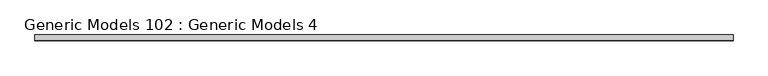
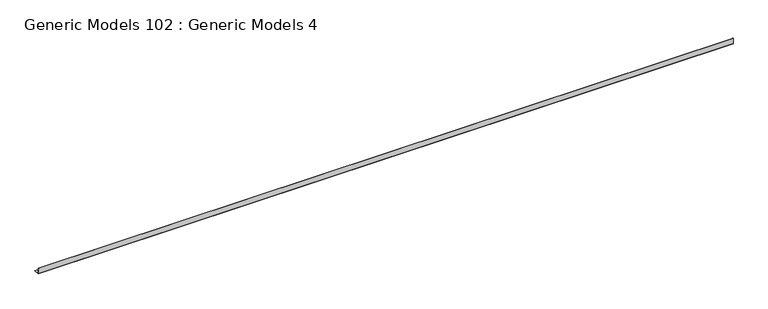
"""IFC4 building model written with IfcOpenShell, lengths in millimetres: proxy geometry, Generic Models 102 : Generic Models 4."""

import ifcopenshell
import ifcopenshell.guid

model = None  # the IFC model being written
_history = None  # IfcOwnerHistory: only IFC2X3 demands one
_inside = {}  # id of a spatial element -> (the spatial element, [elements in it])
_under = {}  # id of a project, library or spatial element -> (it, [spatial elements below it])
_declared = {}  # id of a project -> (the project, [libraries it declares])
_typed = {}  # id of a type object -> (the type object, [elements of that type])
_made_of = {}  # id of a material, layer set ... -> (it, [elements and type objects made of it])


def new_model(schema):
    """Start an empty IFC model of exactly this schema.

    Asked for "IFC4X3", IfcOpenShell would pick the latest addendum, in which some entities
    have other attributes; the version numbers below select the first issue.
    IFC2X3 requires an IfcOwnerHistory on every rooted entity: one is made here for all.
    """
    global model, _history
    if schema == "IFC4X3":
        model = ifcopenshell.file(schema_version=(4, 3, 0, 0))
    else:
        model = ifcopenshell.file(schema=schema)
    _inside.clear()
    _under.clear()
    _declared.clear()
    _typed.clear()
    _made_of.clear()
    _history = None
    if model.schema == "IFC2X3":
        org = make("IfcOrganization", Name="unknown")
        user = make(
            "IfcPersonAndOrganization",
            ThePerson=make("IfcPerson", FamilyName="unknown"),
            TheOrganization=org,
        )
        app = make(
            "IfcApplication",
            ApplicationDeveloper=org,
            Version="unknown",
            ApplicationFullName="unknown",
            ApplicationIdentifier="unknown",
        )
        _history = make(
            "IfcOwnerHistory",
            OwningUser=user,
            OwningApplication=app,
            ChangeAction="ADDED",
            CreationDate=0,
        )
    return model


def make(cls, **values):
    """One entity of the class cls with the attributes given. An attribute that is None is left unset."""
    return model.create_entity(
        cls, **{name: value for name, value in values.items() if value is not None}
    )


def rooted(cls, **values):
    """An entity with a GlobalId (a new one), such as an element, a storey or a relation."""
    return make(cls, GlobalId=ifcopenshell.guid.new(), OwnerHistory=_history, **values)


def si_unit(unit_type, name, prefix=None):
    """IfcSIUnit, for example si_unit("LENGTHUNIT", "METRE", prefix="MILLI")."""
    return make("IfcSIUnit", UnitType=unit_type, Prefix=prefix, Name=name)


def assignment(units):
    """IfcUnitAssignment: the units of a project."""
    return None if units is None else make("IfcUnitAssignment", Units=units)


def point(xyz):
    """IfcCartesianPoint."""
    return None if xyz is None else make("IfcCartesianPoint", Coordinates=xyz)


def direction(xyz):
    """IfcDirection."""
    return None if xyz is None else make("IfcDirection", DirectionRatios=xyz)


def frame(location, z_axis=None, x_axis=None):
    """IfcAxis2Placement3D, a coordinate frame: its origin and axes. An axis left out is left unset."""
    return make(
        "IfcAxis2Placement3D",
        Location=point(location),
        Axis=direction(z_axis),
        RefDirection=direction(x_axis),
    )


def origin():
    """The frame at (0, 0, 0) with its axes left unset."""
    return frame((0.0, 0.0, 0.0))


def place(relative_to, where):
    """IfcLocalPlacement: puts the frame where relative to a parent placement (None: the world)."""
    return make(
        "IfcLocalPlacement", PlacementRelTo=relative_to, RelativePlacement=where
    )


def context(
    kind, dimensions, precision=None, world=None, true_north=None, identifier=None
):
    """IfcGeometricRepresentationContext, for example the 3D "Model" context."""
    return make(
        "IfcGeometricRepresentationContext",
        ContextIdentifier=identifier,
        ContextType=kind,
        CoordinateSpaceDimension=dimensions,
        Precision=precision,
        WorldCoordinateSystem=world,
        TrueNorth=true_north,
    )


def project(units=None, contexts=None):
    """IfcProject with its units and contexts."""
    return rooted(
        "IfcProject",
        Name="project",
        RepresentationContexts=contexts,
        UnitsInContext=assignment(units),
    )


def spatial(cls, under=None, at=None, **own):
    """A site, building, storey or space (cls), placed at a placement, below another one or the project."""
    s = rooted(cls, ObjectPlacement=at, **own)
    if under is not None:
        _under.setdefault(under.id(), (under, []))[1].append(s)
    return s


def polyline(points):
    """IfcPolyline through the points."""
    return make("IfcPolyline", Points=[point(p) for p in points])


def outline(outer, holes=None, kind="AREA"):
    """IfcArbitraryClosedProfileDef: a profile drawn as a closed curve; with holes, ...WithVoids."""
    if holes is None:
        return make("IfcArbitraryClosedProfileDef", ProfileType=kind, OuterCurve=outer)
    return make(
        "IfcArbitraryProfileDefWithVoids",
        ProfileType=kind,
        OuterCurve=outer,
        InnerCurves=holes,
    )


def extrude(swept, where, along, depth):
    """IfcExtrudedAreaSolid: the profile swept, set in the frame where, extruded along a direction by depth."""
    return make(
        "IfcExtrudedAreaSolid",
        SweptArea=swept,
        Position=where,
        ExtrudedDirection=direction(along),
        Depth=depth,
    )


def shape(context_of_items, identifier, shape_type, items):
    """IfcShapeRepresentation: the items that make up one representation, for example the "Body"."""
    return make(
        "IfcShapeRepresentation",
        ContextOfItems=context_of_items,
        RepresentationIdentifier=identifier,
        RepresentationType=shape_type,
        Items=items,
    )


def source(mapping_origin, context_of_items, identifier, shape_type, items):
    """IfcRepresentationMap: a shape defined once, which mapped items show again and again."""
    return make(
        "IfcRepresentationMap",
        MappingOrigin=mapping_origin,
        MappedRepresentation=shape(context_of_items, identifier, shape_type, items),
    )


def transform(
    local_origin,
    x_axis=None,
    y_axis=None,
    z_axis=None,
    scale=None,
    scale2=None,
    scale3=None,
    uniform=True,
):
    """IfcCartesianTransformationOperator3D, or its non-uniform kind. x_axis, y_axis, z_axis: its Axis1, 2, 3."""
    if uniform:
        return make(
            "IfcCartesianTransformationOperator3D",
            Axis1=direction(x_axis),
            Axis2=direction(y_axis),
            LocalOrigin=point(local_origin),
            Scale=scale,
            Axis3=direction(z_axis),
        )
    return make(
        "IfcCartesianTransformationOperator3DnonUniform",
        Axis1=direction(x_axis),
        Axis2=direction(y_axis),
        LocalOrigin=point(local_origin),
        Scale=scale,
        Axis3=direction(z_axis),
        Scale2=scale2,
        Scale3=scale3,
    )


def mapped(mapping_source, mapping_target):
    """IfcMappedItem: shows the shape of a source again, moved by a transform."""
    return make(
        "IfcMappedItem", MappingSource=mapping_source, MappingTarget=mapping_target
    )


def made_of(thing, what):
    """Note that an element or type object is made of a material, layer set ...; save() writes the relation."""
    if what is not None:
        _made_of.setdefault(what.id(), (what, []))[1].append(thing)
    return thing


def element(
    cls,
    number,
    at=None,
    inside=None,
    cuts=None,
    type_object=None,
    material=None,
    context=None,
    identifier="Body",
    shape_type=None,
    held_by="IfcProductDefinitionShape",
    body=None,
    shapes=None,
    **own,
):
    """One element of the class cls, such as IfcWall. Its Tag is "e" and its number.

    at: its placement. inside: the storey or other place that contains it. cuts: it is an
    opening in that element (IfcRelVoidsElement). A single representation is given by context,
    identifier, shape_type and body (its items); several are given by shapes. held_by: the class
    of the entity that holds the representations. save() writes the other relations.
    """
    e = rooted(cls, Tag="e%d" % number, ObjectPlacement=at, **own)
    if body is not None:
        shapes = [shape(context, identifier, shape_type, body)]
    if shapes is not None:
        e.Representation = make(held_by, Representations=shapes)
    if inside is not None:
        _inside.setdefault(inside.id(), (inside, []))[1].append(e)
    if cuts is not None:
        rooted(
            "IfcRelVoidsElement", RelatingBuildingElement=cuts, RelatedOpeningElement=e
        )
    if type_object is not None:
        _typed.setdefault(type_object.id(), (type_object, []))[1].append(e)
    return made_of(e, material)


def aggregate(whole, parts):
    """IfcRelAggregates: a whole, such as a stair, and the parts it consists of."""
    return rooted("IfcRelAggregates", RelatingObject=whole, RelatedObjects=parts)


def save(model, path):
    """Write the relations noted so far, then the file.

    IfcRelAggregates (storeys below a building ...), IfcRelContainedInSpatialStructure (elements
    in a storey), IfcRelDefinesByType, IfcRelAssociatesMaterial and IfcRelDeclares: one each for
    every whole, place, type object, material and project.
    """
    for whole, parts in _under.values():
        aggregate(whole, parts)
    for where, things in _inside.values():
        rooted(
            "IfcRelContainedInSpatialStructure",
            RelatedElements=things,
            RelatingStructure=where,
        )
    for kind, things in _typed.values():
        rooted("IfcRelDefinesByType", RelatedObjects=things, RelatingType=kind)
    for what, things in _made_of.values():
        rooted("IfcRelAssociatesMaterial", RelatedObjects=things, RelatingMaterial=what)
    for by, libraries in _declared.values():
        rooted("IfcRelDeclares", RelatingContext=by, RelatedDefinitions=libraries)
    model.write(path)


def generic_models_102_generic_models_4_adb4bbdb(model_context):
    return source(origin(), model_context, "Body", "SweptSolid", [
        extrude(outline(polyline([(7055.9241645, 126940.7261365), (7208.2911024, 126937.5518253), (7208.2745695, 126936.7582475), (7055.1304145, 126939.9487507), (7055.1304145, 127093.1261365), (7055.9241645, 127093.1261365), (7055.9241645, 126940.7261365)])), frame((-10234.5171316, 0.0, 0.0), z_axis=(1.0, 0.0, 0.0), x_axis=(0.0, 1.0, 0.0)), (0.0, 0.0, 1.0), 18643.6),
    ])


if __name__ == "__main__":
    model = new_model("IFC4")
    model_context = context("Model", 3, world=origin())
    ifc_project = project(units=[si_unit("LENGTHUNIT", "METRE", prefix="MILLI")], contexts=[model_context])
    site = spatial("IfcSite", under=ifc_project)
    building = spatial("IfcBuilding", under=site)
    placement = place(None, origin())
    generic_models_102_generic_models_4_shape = generic_models_102_generic_models_4_adb4bbdb(model_context)
    element("IfcBuildingElementProxy", 1, Name="Generic Models 102 : Generic Models 4", ObjectType="Generic Models 102 : Generic Models 4", at=placement, inside=building, context=model_context, shape_type="MappedRepresentation", body=[
        mapped(generic_models_102_generic_models_4_shape, transform((0.0, 0.0, 0.0), x_axis=(1.0, 0.0, 0.0), y_axis=(0.0, 1.0, 0.0), z_axis=(0.0, 0.0, 1.0))),
    ])
    save(model, "model.ifc")

# Revit data of these elements
# Element 1 (IfcBuildingElementProxy, "Generic Models 102 : Generic Models 4")
#   Materials on its faces: "_16 GA. COPPER \"L\" FLASHING - (6\" HORZ. LEG - 4\" VERT. LEG)"
# Materials
#   "_16 GA. COPPER \"L\" FLASHING - (6\" HORZ. LEG - 4\" VERT. LEG)": class "Generic", colour RGB 156 184 169, transparency 0, Cost = 0
